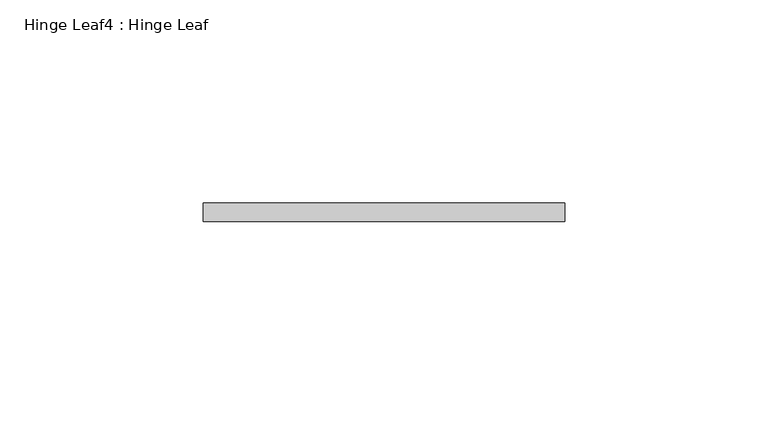
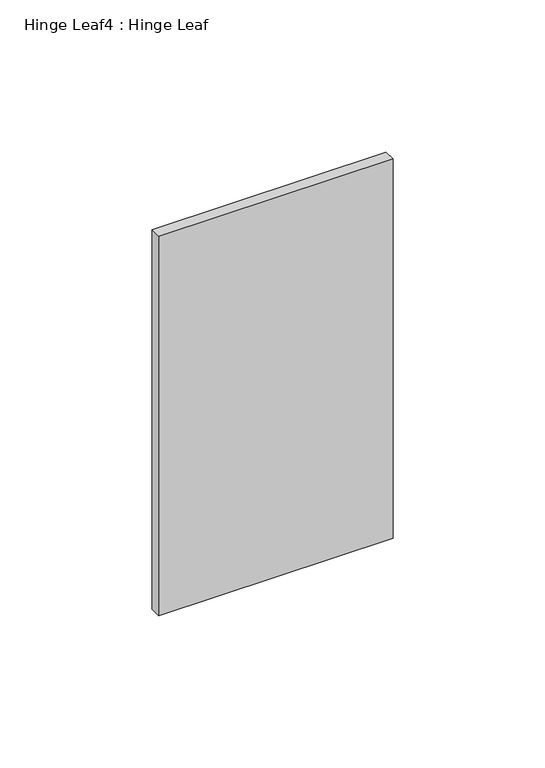
"""IFC4 building model written with IfcOpenShell, lengths in millimetres: proxy geometry, Hinge Leaf4 : Hinge Leaf."""

from ifc_helpers import new_model, si_unit, frame, origin, place, context, project, spatial, polyline, outline, extrude, source, transform, mapped, element, save


def hinge_leaf4_hinge_leaf_dc6140c5(model_context):
    return source(origin(), model_context, "Body", "SweptSolid", [
        extrude(outline(polyline([(587327.7934739, -531780.6943841), (587416.6934739, -531780.6943841), (587416.6934739, -531785.2663841), (587327.7934739, -531785.2663841), (587327.7934739, -531780.6943841)])), frame((0.0, 0.0, 1936.75), z_axis=(0.0, 0.0, 1.0), x_axis=(1.0, 0.0, 0.0)), (0.0, 0.0, 1.0), 152.4),
    ])


if __name__ == "__main__":
    model = new_model("IFC4")
    model_context = context("Model", 3, world=origin())
    ifc_project = project(units=[si_unit("LENGTHUNIT", "METRE", prefix="MILLI")], contexts=[model_context])
    site = spatial("IfcSite", under=ifc_project)
    building = spatial("IfcBuilding", under=site)
    placement = place(None, origin())
    hinge_leaf4_hinge_leaf_shape = hinge_leaf4_hinge_leaf_dc6140c5(model_context)
    element("IfcBuildingElementProxy", 1, Name="Hinge Leaf4 : Hinge Leaf", ObjectType="Hinge Leaf4 : Hinge Leaf", at=placement, inside=building, context=model_context, shape_type="MappedRepresentation", body=[
        mapped(hinge_leaf4_hinge_leaf_shape, transform((0.0, 0.0, 0.0), x_axis=(1.0, 0.0, 0.0), y_axis=(0.0, 1.0, 0.0), z_axis=(0.0, 0.0, 1.0))),
    ])
    save(model, "model.ifc")

# Revit data of these elements
# Element 1 (IfcBuildingElementProxy, "Hinge Leaf4 : Hinge Leaf")
#   Materials on its faces: "6\"X6\" WELD-ON STL BUTT HINGE"
# Materials
#   "6\"X6\" WELD-ON STL BUTT HINGE": class "Metal", colour RGB 189 187 185, transparency 0, Description = "Carbon steel", Cost = 0
